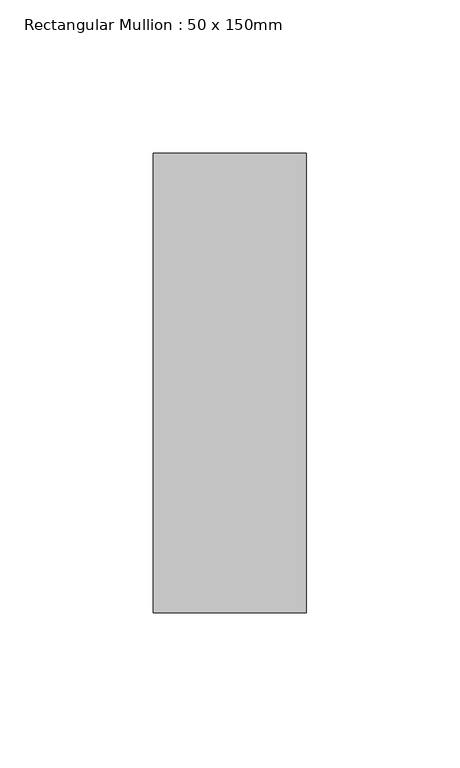
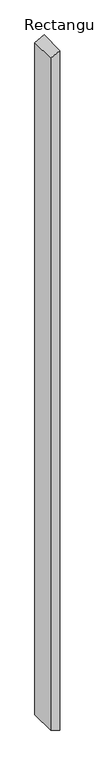
"""IFC4 building model written with IfcOpenShell, lengths in millimetres: member geometry, Rectangular Mullion : 50 x 150mm."""

from ifc_helpers import new_model, si_unit, frame, origin, place, context, project, spatial, polyline, outline, extrude, source, transform, mapped, element, save


def rectangular_mullion_50_x_150mm_8c2aeeaa(model_context):
    return source(origin(), model_context, "Body", "SweptSolid", [
        extrude(outline(polyline([(0.0, 0.0), (-26.9507667, -50.0), (-3926.5430895, -50.0), (-3943.1772756, 0.0), (0.0, 0.0)])), frame((0.0, -75.0, 0.0), z_axis=(0.0, 1.0, 0.0), x_axis=(0.0, 0.0, 1.0)), (0.0, 0.0, 1.0), 150.0),
    ])


if __name__ == "__main__":
    model = new_model("IFC4")
    model_context = context("Model", 3, world=origin())
    ifc_project = project(units=[si_unit("LENGTHUNIT", "METRE", prefix="MILLI")], contexts=[model_context])
    site = spatial("IfcSite", under=ifc_project)
    building = spatial("IfcBuilding", under=site)
    placement = place(None, origin())
    rectangular_mullion_50_x_150mm_shape = rectangular_mullion_50_x_150mm_8c2aeeaa(model_context)
    element("IfcMember", 1, ObjectType="Rectangular Mullion : 50 x 150mm", at=placement, inside=building, context=model_context, shape_type="MappedRepresentation", body=[
        mapped(rectangular_mullion_50_x_150mm_shape, transform((0.0, 0.0, 0.0), x_axis=(1.0, 0.0, 0.0), y_axis=(0.0, 1.0, 0.0), z_axis=(0.0, 0.0, 1.0))),
    ])
    save(model, "model.ifc")

# Revit data of these elements
# Type "Rectangular Mullion : 50 x 150mm"
#   built-in parameter 1007304 = 0.492126 (stored number, unit not read)
#   built-in parameter 1007301 = 0.082021 (stored number, unit not read)
#   built-in parameter 1007300 = 0.082021 (stored number, unit not read)
# Element 1 (IfcMember, "Rectangular Mullion : 50 x 150mm")
#   Materials on its faces: "Metal - Aluminium"
# Materials
#   "Metal - Aluminium": class "Metal", colour RGB 247 247 247, transparency 0
